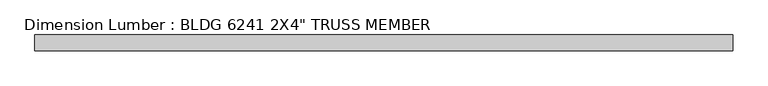
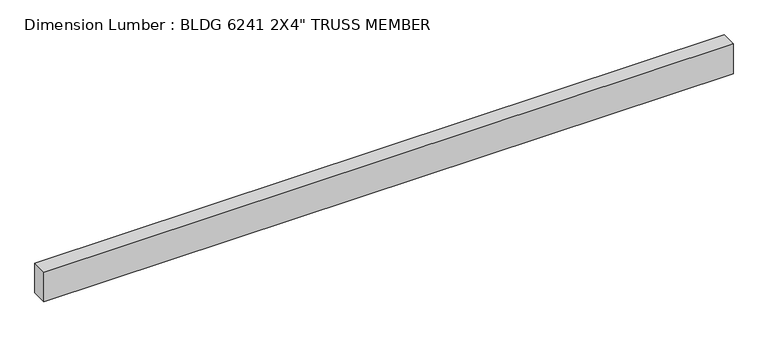
"""IFC4 building model written with IfcOpenShell, lengths in millimetres: beam geometry."""

import ifcopenshell
import ifcopenshell.guid

model = None  # the IFC model being written
_history = None  # IfcOwnerHistory: only IFC2X3 demands one
_inside = {}  # id of a spatial element -> (the spatial element, [elements in it])
_under = {}  # id of a project, library or spatial element -> (it, [spatial elements below it])
_declared = {}  # id of a project -> (the project, [libraries it declares])
_typed = {}  # id of a type object -> (the type object, [elements of that type])
_made_of = {}  # id of a material, layer set ... -> (it, [elements and type objects made of it])


def new_model(schema):
    """Start an empty IFC model of exactly this schema.

    Asked for "IFC4X3", IfcOpenShell would pick the latest addendum, in which some entities
    have other attributes; the version numbers below select the first issue.
    IFC2X3 requires an IfcOwnerHistory on every rooted entity: one is made here for all.
    """
    global model, _history
    if schema == "IFC4X3":
        model = ifcopenshell.file(schema_version=(4, 3, 0, 0))
    else:
        model = ifcopenshell.file(schema=schema)
    _inside.clear()
    _under.clear()
    _declared.clear()
    _typed.clear()
    _made_of.clear()
    _history = None
    if model.schema == "IFC2X3":
        org = make("IfcOrganization", Name="unknown")
        user = make(
            "IfcPersonAndOrganization",
            ThePerson=make("IfcPerson", FamilyName="unknown"),
            TheOrganization=org,
        )
        app = make(
            "IfcApplication",
            ApplicationDeveloper=org,
            Version="unknown",
            ApplicationFullName="unknown",
            ApplicationIdentifier="unknown",
        )
        _history = make(
            "IfcOwnerHistory",
            OwningUser=user,
            OwningApplication=app,
            ChangeAction="ADDED",
            CreationDate=0,
        )
    return model


def make(cls, **values):
    """One entity of the class cls with the attributes given. An attribute that is None is left unset."""
    return model.create_entity(
        cls, **{name: value for name, value in values.items() if value is not None}
    )


def rooted(cls, **values):
    """An entity with a GlobalId (a new one), such as an element, a storey or a relation."""
    return make(cls, GlobalId=ifcopenshell.guid.new(), OwnerHistory=_history, **values)


def si_unit(unit_type, name, prefix=None):
    """IfcSIUnit, for example si_unit("LENGTHUNIT", "METRE", prefix="MILLI")."""
    return make("IfcSIUnit", UnitType=unit_type, Prefix=prefix, Name=name)


def assignment(units):
    """IfcUnitAssignment: the units of a project."""
    return None if units is None else make("IfcUnitAssignment", Units=units)


def point(xyz):
    """IfcCartesianPoint."""
    return None if xyz is None else make("IfcCartesianPoint", Coordinates=xyz)


def direction(xyz):
    """IfcDirection."""
    return None if xyz is None else make("IfcDirection", DirectionRatios=xyz)


def frame(location, z_axis=None, x_axis=None):
    """IfcAxis2Placement3D, a coordinate frame: its origin and axes. An axis left out is left unset."""
    return make(
        "IfcAxis2Placement3D",
        Location=point(location),
        Axis=direction(z_axis),
        RefDirection=direction(x_axis),
    )


def origin():
    """The frame at (0, 0, 0) with its axes left unset."""
    return frame((0.0, 0.0, 0.0))


def place(relative_to, where):
    """IfcLocalPlacement: puts the frame where relative to a parent placement (None: the world)."""
    return make(
        "IfcLocalPlacement", PlacementRelTo=relative_to, RelativePlacement=where
    )


def context(
    kind, dimensions, precision=None, world=None, true_north=None, identifier=None
):
    """IfcGeometricRepresentationContext, for example the 3D "Model" context."""
    return make(
        "IfcGeometricRepresentationContext",
        ContextIdentifier=identifier,
        ContextType=kind,
        CoordinateSpaceDimension=dimensions,
        Precision=precision,
        WorldCoordinateSystem=world,
        TrueNorth=true_north,
    )


def project(units=None, contexts=None):
    """IfcProject with its units and contexts."""
    return rooted(
        "IfcProject",
        Name="project",
        RepresentationContexts=contexts,
        UnitsInContext=assignment(units),
    )


def spatial(cls, under=None, at=None, **own):
    """A site, building, storey or space (cls), placed at a placement, below another one or the project."""
    s = rooted(cls, ObjectPlacement=at, **own)
    if under is not None:
        _under.setdefault(under.id(), (under, []))[1].append(s)
    return s


def polyline(points):
    """IfcPolyline through the points."""
    return make("IfcPolyline", Points=[point(p) for p in points])


def outline(outer, holes=None, kind="AREA"):
    """IfcArbitraryClosedProfileDef: a profile drawn as a closed curve; with holes, ...WithVoids."""
    if holes is None:
        return make("IfcArbitraryClosedProfileDef", ProfileType=kind, OuterCurve=outer)
    return make(
        "IfcArbitraryProfileDefWithVoids",
        ProfileType=kind,
        OuterCurve=outer,
        InnerCurves=holes,
    )


def extrude(swept, where, along, depth):
    """IfcExtrudedAreaSolid: the profile swept, set in the frame where, extruded along a direction by depth."""
    return make(
        "IfcExtrudedAreaSolid",
        SweptArea=swept,
        Position=where,
        ExtrudedDirection=direction(along),
        Depth=depth,
    )


def shape(context_of_items, identifier, shape_type, items):
    """IfcShapeRepresentation: the items that make up one representation, for example the "Body"."""
    return make(
        "IfcShapeRepresentation",
        ContextOfItems=context_of_items,
        RepresentationIdentifier=identifier,
        RepresentationType=shape_type,
        Items=items,
    )


def source(mapping_origin, context_of_items, identifier, shape_type, items):
    """IfcRepresentationMap: a shape defined once, which mapped items show again and again."""
    return make(
        "IfcRepresentationMap",
        MappingOrigin=mapping_origin,
        MappedRepresentation=shape(context_of_items, identifier, shape_type, items),
    )


def transform(
    local_origin,
    x_axis=None,
    y_axis=None,
    z_axis=None,
    scale=None,
    scale2=None,
    scale3=None,
    uniform=True,
):
    """IfcCartesianTransformationOperator3D, or its non-uniform kind. x_axis, y_axis, z_axis: its Axis1, 2, 3."""
    if uniform:
        return make(
            "IfcCartesianTransformationOperator3D",
            Axis1=direction(x_axis),
            Axis2=direction(y_axis),
            LocalOrigin=point(local_origin),
            Scale=scale,
            Axis3=direction(z_axis),
        )
    return make(
        "IfcCartesianTransformationOperator3DnonUniform",
        Axis1=direction(x_axis),
        Axis2=direction(y_axis),
        LocalOrigin=point(local_origin),
        Scale=scale,
        Axis3=direction(z_axis),
        Scale2=scale2,
        Scale3=scale3,
    )


def mapped(mapping_source, mapping_target):
    """IfcMappedItem: shows the shape of a source again, moved by a transform."""
    return make(
        "IfcMappedItem", MappingSource=mapping_source, MappingTarget=mapping_target
    )


def made_of(thing, what):
    """Note that an element or type object is made of a material, layer set ...; save() writes the relation."""
    if what is not None:
        _made_of.setdefault(what.id(), (what, []))[1].append(thing)
    return thing


def element(
    cls,
    number,
    at=None,
    inside=None,
    cuts=None,
    type_object=None,
    material=None,
    context=None,
    identifier="Body",
    shape_type=None,
    held_by="IfcProductDefinitionShape",
    body=None,
    shapes=None,
    **own,
):
    """One element of the class cls, such as IfcWall. Its Tag is "e" and its number.

    at: its placement. inside: the storey or other place that contains it. cuts: it is an
    opening in that element (IfcRelVoidsElement). A single representation is given by context,
    identifier, shape_type and body (its items); several are given by shapes. held_by: the class
    of the entity that holds the representations. save() writes the other relations.
    """
    e = rooted(cls, Tag="e%d" % number, ObjectPlacement=at, **own)
    if body is not None:
        shapes = [shape(context, identifier, shape_type, body)]
    if shapes is not None:
        e.Representation = make(held_by, Representations=shapes)
    if inside is not None:
        _inside.setdefault(inside.id(), (inside, []))[1].append(e)
    if cuts is not None:
        rooted(
            "IfcRelVoidsElement", RelatingBuildingElement=cuts, RelatedOpeningElement=e
        )
    if type_object is not None:
        _typed.setdefault(type_object.id(), (type_object, []))[1].append(e)
    return made_of(e, material)


def aggregate(whole, parts):
    """IfcRelAggregates: a whole, such as a stair, and the parts it consists of."""
    return rooted("IfcRelAggregates", RelatingObject=whole, RelatedObjects=parts)


def save(model, path):
    """Write the relations noted so far, then the file.

    IfcRelAggregates (storeys below a building ...), IfcRelContainedInSpatialStructure (elements
    in a storey), IfcRelDefinesByType, IfcRelAssociatesMaterial and IfcRelDeclares: one each for
    every whole, place, type object, material and project.
    """
    for whole, parts in _under.values():
        aggregate(whole, parts)
    for where, things in _inside.values():
        rooted(
            "IfcRelContainedInSpatialStructure",
            RelatedElements=things,
            RelatingStructure=where,
        )
    for kind, things in _typed.values():
        rooted("IfcRelDefinesByType", RelatedObjects=things, RelatingType=kind)
    for what, things in _made_of.values():
        rooted("IfcRelAssociatesMaterial", RelatedObjects=things, RelatingMaterial=what)
    for by, libraries in _declared.values():
        rooted("IfcRelDeclares", RelatingContext=by, RelatedDefinitions=libraries)
    model.write(path)


def beam_50604119(model_context):
    return source(origin(), model_context, "Body", "SweptSolid", [
        extrude(outline(polyline([(1117.6, 25.4), (1117.6, -25.4), (-1117.6, -25.4), (-1117.6, 25.4), (1117.6, 25.4)])), frame((0.0, 0.0, -50.8), z_axis=(0.0, 0.0, 1.0), x_axis=(1.0, 0.0, 0.0)), (0.0, 0.0, 1.0), 101.6),
    ])


if __name__ == "__main__":
    model = new_model("IFC4")
    model_context = context("Model", 3, world=origin())
    ifc_project = project(units=[si_unit("LENGTHUNIT", "METRE", prefix="MILLI")], contexts=[model_context])
    site = spatial("IfcSite", under=ifc_project)
    building = spatial("IfcBuilding", under=site)
    placement = place(None, origin())
    beam_shape = beam_50604119(model_context)
    element("IfcBeam", 1, ObjectType="Dimension Lumber : BLDG 6241 2X4\" TRUSS MEMBER", at=placement, inside=building, context=model_context, shape_type="MappedRepresentation", body=[
        mapped(beam_shape, transform((0.0, 0.0, 0.0), x_axis=(1.0, 0.0, 0.0), y_axis=(0.0, 1.0, 0.0), z_axis=(0.0, 0.0, 1.0))),
    ])
    save(model, "model.ifc")

# Revit data of these elements
# Type "Dimension Lumber : BLDG 6241 2X4\" TRUSS MEMBER"
#   Assembly Code = "B10"
#   A = 0.273472 SF
#   Length [instance default] = 5' - 0"
#   b = 0' - 2"
#   d = 0' - 4"
#   Structural Material [instance default] = Softwood, Lumber
# Element 1 (IfcBeam, "Dimension Lumber : BLDG 6241 2X4\" TRUSS MEMBER")
#   Materials on its faces: "Softwood, Lumber"
# Materials
#   "Softwood, Lumber": class "Wood", colour RGB 223 192 134, transparency 0, Description = "Pinus Echinata", Cost = 0
